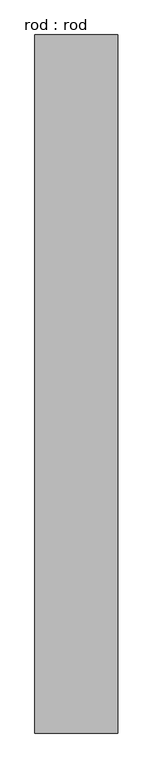
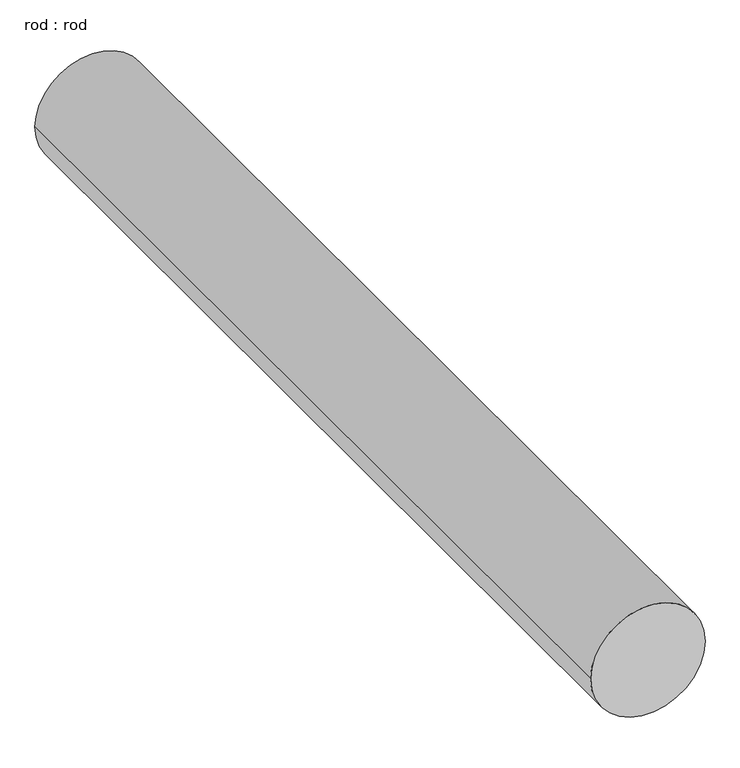
"""IFC4 building model written with IfcOpenShell, lengths in millimetres: proxy geometry, rod : rod."""

from ifc_helpers import new_model, si_unit, point, frame, frame_2d, origin, place, context, project, spatial, circle_curve, trimmed, segment, composite_curve, outline, extrude, source, transform, mapped, element, save


def rod_rod_d6a5075f(model_context):
    return source(origin(), model_context, "Body", "SweptSolid", [
        extrude(outline(composite_curve([segment(trimmed(circle_curve(frame_2d((0.0108462, 0.0)), 200.0), [point((0.0108462, 200.0))], [point((0.0108462, -200.0))], False, "CARTESIAN"), True, "CONTINUOUS"), segment(trimmed(circle_curve(frame_2d((0.0108462, 0.0)), 200.0), [point((0.0108462, -200.0))], [point((0.0108462, 200.0))], False, "CARTESIAN"), True, "CONTINUOUS")], self_intersect=False)), frame((0.0, 2410.5857582, 0.0), z_axis=(0.0, 1.0, 0.0), x_axis=(0.0, 0.0, 1.0)), (0.0, 0.0, 1.0), 3364.2857143),
    ])


if __name__ == "__main__":
    model = new_model("IFC4")
    model_context = context("Model", 3, world=origin())
    ifc_project = project(units=[si_unit("LENGTHUNIT", "METRE", prefix="MILLI")], contexts=[model_context])
    site = spatial("IfcSite", under=ifc_project)
    building = spatial("IfcBuilding", under=site)
    placement = place(None, origin())
    rod_rod_shape = rod_rod_d6a5075f(model_context)
    element("IfcBuildingElementProxy", 1, Name="rod : rod", ObjectType="rod : rod", at=placement, inside=building, context=model_context, shape_type="MappedRepresentation", body=[
        mapped(rod_rod_shape, transform((0.0, 0.0, 0.0), x_axis=(1.0, 0.0, 0.0), y_axis=(0.0, 1.0, 0.0), z_axis=(0.0, 0.0, 1.0))),
    ])
    save(model, "model.ifc")

# Revit data of these elements
# Type "rod : rod"
#   Default Elevation = 0
